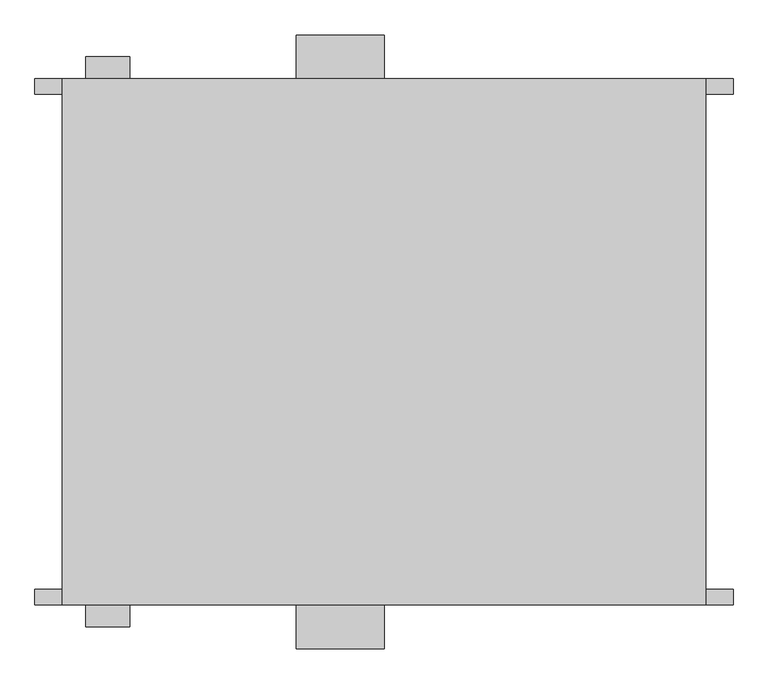
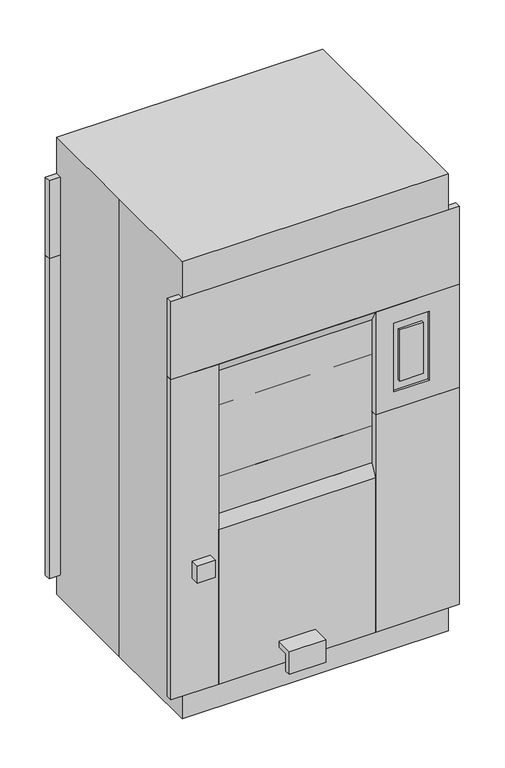
"""IFC4 building model written with IfcOpenShell, lengths in millimetres: proxy geometry, S0960 - Washer-Disinfector, STM, 2 DO, RCSD1WLL, 26x24x24 Cham : S0960 - Washer-Disinfector, STM, 2 DO, RCSD1WLL, 26x24x24 Cham."""

from ifc_helpers import new_model, si_unit, frame, origin, place, context, project, spatial, polyline, outline, extrude, faceted_brep, source, transform, mapped, element, save


def specialty_equipment_aeb0d0a3(model_context):
    return source(origin(), model_context, "Body", "SolidModel", [
        extrude(outline(polyline([(-457.2, 101.6), (-457.2, 787.4), (-430.2125, 838.2), (-430.2125, 101.6), (-457.2, 101.6)])), frame((-406.4, 0.0, 0.0), z_axis=(1.0, 0.0, 0.0), x_axis=(0.0, 1.0, 0.0)), (0.0, 0.0, 1.0), 660.4),
        extrude(outline(polyline([(-430.2125, 1524.0), (-430.2125, 1473.2), (-457.2, 1524.0), (-430.2125, 1524.0)])), frame((-406.4, 0.0, 0.0), z_axis=(1.0, 0.0, 0.0), x_axis=(0.0, 1.0, 0.0)), (0.0, 0.0, 1.0), 660.4),
        faceted_brep([(606.425, -457.2, 1524.0), (254.0, -457.2, 1524.0), (254.0, -457.2, 1066.8), (606.425, -457.2, 1066.8), (479.425, -457.2, 1447.8), (479.425, -457.2, 1143.0), (330.2, -457.2, 1143.0), (330.2, -457.2, 1447.8), (454.025, -457.2, 1409.7), (355.6, -457.2, 1409.7), (355.6, -457.2, 1181.1), (454.025, -457.2, 1181.1), (606.425, -430.2125, 1524.0), (606.425, -430.2125, 1066.8), (254.0, -430.2125, 1066.8), (254.0, -430.2125, 1524.0), (479.425, -448.0871048, 1447.8), (330.2, -448.0871048, 1447.8), (330.2, -448.0871048, 1143.0), (479.425, -448.0871048, 1143.0), (454.025, -448.0871048, 1409.7), (454.025, -448.0871048, 1181.1), (355.6, -448.0871048, 1181.1), (355.6, -448.0871048, 1409.7)], [[[0, 1, 2, 3], [4, 5, 6, 7]], [[8, 9, 10, 11]], [[12, 13, 14, 15]], [[0, 12, 15, 1]], [[1, 15, 14, 2]], [[2, 14, 13, 3]], [[3, 13, 12, 0]], [[16, 17, 18, 19], [20, 21, 22, 23]], [[16, 4, 7, 17]], [[17, 7, 6, 18]], [[18, 6, 5, 19]], [[19, 5, 4, 16]], [[20, 8, 11, 21]], [[21, 11, 10, 22]], [[22, 10, 9, 23]], [[23, 9, 8, 20]]]),
        extrude(outline(polyline([(606.425, 457.2), (606.425, 430.2125), (254.0, 430.2125), (254.0, 457.2), (606.425, 457.2)])), frame((0.0, 0.0, 101.6), z_axis=(0.0, 0.0, 1.0), x_axis=(1.0, 0.0, 0.0)), (0.0, 0.0, 1.0), 965.2),
        extrude(outline(polyline([(-406.4, 457.2), (-406.4, 430.2125), (-606.425, 430.2125), (-606.425, 457.2), (-406.4, 457.2)])), frame((0.0, 0.0, 101.6), z_axis=(0.0, 0.0, 1.0), x_axis=(1.0, 0.0, 0.0)), (0.0, 0.0, 1.0), 1422.4),
        extrude(outline(polyline([(606.425, 457.2), (606.425, 430.2125), (-606.425, 430.2125), (-606.425, 457.2), (606.425, 457.2)])), frame((0.0, 0.0, 1524.0), z_axis=(0.0, 0.0, 1.0), x_axis=(1.0, 0.0, 0.0)), (0.0, 0.0, 1.0), 346.075),
        extrude(outline(polyline([(-533.4, 203.2), (-457.2, 203.2), (-457.2, 177.8), (-508.0, 177.8), (-508.0, 101.6), (-533.4, 101.6), (-533.4, 203.2)])), frame((-152.4, 0.0, 0.0), z_axis=(1.0, 0.0, 0.0), x_axis=(0.0, 1.0, 0.0)), (0.0, 0.0, 1.0), 152.4),
        extrude(outline(polyline([(-517.7182221, -495.3), (-517.7182221, -457.2), (-441.5182221, -457.2), (-441.5182221, -495.3), (-517.7182221, -495.3)])), frame((0.0, 0.0, 611.2734951), z_axis=(0.0, 0.0, 1.0), x_axis=(1.0, 0.0, 0.0)), (0.0, 0.0, 1.0), 76.2),
        extrude(outline(polyline([(254.0, -457.2), (254.0, -430.2125), (606.425, -430.2125), (606.425, -457.2), (254.0, -457.2)])), frame((0.0, 0.0, 101.6), z_axis=(0.0, 0.0, 1.0), x_axis=(1.0, 0.0, 0.0)), (0.0, 0.0, 1.0), 965.2),
        extrude(outline(polyline([(-606.425, -457.2), (-606.425, -430.2125), (-406.4, -430.2125), (-406.4, -457.2), (-606.425, -457.2)])), frame((0.0, 0.0, 101.6), z_axis=(0.0, 0.0, 1.0), x_axis=(1.0, 0.0, 0.0)), (0.0, 0.0, 1.0), 1422.4),
        extrude(outline(polyline([(-606.425, -457.2), (-606.425, -430.2125), (606.425, -430.2125), (606.425, -457.2), (-606.425, -457.2)])), frame((0.0, 0.0, 1524.0), z_axis=(0.0, 0.0, 1.0), x_axis=(1.0, 0.0, 0.0)), (0.0, 0.0, 1.0), 346.075),
        extrude(outline(polyline([(533.4, 203.2), (533.4, 101.6), (508.0, 101.6), (508.0, 177.8), (457.2, 177.8), (457.2, 203.2), (533.4, 203.2)])), frame((-152.4, 0.0, 0.0), z_axis=(1.0, 0.0, 0.0), x_axis=(0.0, 1.0, 0.0)), (0.0, 0.0, 1.0), 152.4),
        extrude(outline(polyline([(-441.5182221, 495.3), (-441.5182221, 457.2), (-517.7182221, 457.2), (-517.7182221, 495.3), (-441.5182221, 495.3)])), frame((0.0, 0.0, 611.2734951), z_axis=(0.0, 0.0, 1.0), x_axis=(1.0, 0.0, 0.0)), (0.0, 0.0, 1.0), 76.2),
        extrude(outline(polyline([(430.2125, 101.6), (430.2125, 838.2), (457.2, 787.4), (457.2, 101.6), (430.2125, 101.6)])), frame((-406.4, 0.0, 0.0), z_axis=(1.0, 0.0, 0.0), x_axis=(0.0, 1.0, 0.0)), (0.0, 0.0, 1.0), 660.4),
        extrude(outline(polyline([(457.2, 1524.0), (430.2125, 1473.2), (430.2125, 1524.0), (457.2, 1524.0)])), frame((-406.4, 0.0, 0.0), z_axis=(1.0, 0.0, 0.0), x_axis=(0.0, 1.0, 0.0)), (0.0, 0.0, 1.0), 660.4),
        faceted_brep([(606.425, 457.2, 1524.0), (606.425, 457.2, 1066.8), (254.0, 457.2, 1066.8), (254.0, 457.2, 1524.0), (330.2, 457.2, 1447.8), (330.2, 457.2, 1143.0), (479.425, 457.2, 1143.0), (479.425, 457.2, 1447.8), (454.025, 457.2, 1181.1), (355.6, 457.2, 1181.1), (355.6, 457.2, 1409.7), (454.025, 457.2, 1409.7), (606.425, 430.2125, 1524.0), (254.0, 430.2125, 1524.0), (254.0, 430.2125, 1066.8), (606.425, 430.2125, 1066.8), (479.425, 448.0871048, 1447.8), (479.425, 448.0871048, 1143.0), (330.2, 448.0871048, 1143.0), (330.2, 448.0871048, 1447.8), (454.025, 448.0871048, 1409.7), (355.6, 448.0871048, 1409.7), (355.6, 448.0871048, 1181.1), (454.025, 448.0871048, 1181.1)], [[[0, 1, 2, 3], [4, 5, 6, 7]], [[8, 9, 10, 11]], [[12, 13, 14, 15]], [[3, 13, 12, 0]], [[2, 14, 13, 3]], [[1, 15, 14, 2]], [[0, 12, 15, 1]], [[16, 17, 18, 19], [20, 21, 22, 23]], [[19, 4, 7, 16]], [[18, 5, 4, 19]], [[17, 6, 5, 18]], [[16, 7, 6, 17]], [[23, 8, 11, 20]], [[22, 9, 8, 23]], [[21, 10, 9, 22]], [[20, 11, 10, 21]]]),
        extrude(outline(polyline([(254.0, 430.2125), (254.0, -430.2125), (-406.4, -430.2125), (-406.4, 430.2125), (254.0, 430.2125)])), frame((0.0, 0.0, 838.2), z_axis=(0.0, 0.0, 1.0), x_axis=(1.0, 0.0, 0.0)), (0.0, 0.0, 1.0), 635.0),
        extrude(outline(polyline([(0.0, 555.625), (1870.075, 555.625), (1870.075, -555.625), (0.0, -555.625), (0.0, 555.625)]), holes=[polyline([(838.2, -406.4), (996.95, -406.4), (996.95, 254.0), (838.2, 254.0), (838.2, -406.4)]), polyline([(1473.2, 254.0), (1320.8, 254.0), (1320.8, -406.4), (1473.2, -406.4), (1473.2, 254.0)]), polyline([(1314.45, 254.0), (1162.05, 254.0), (1162.05, -406.4), (1314.45, -406.4), (1314.45, 254.0)]), polyline([(1155.7, 254.0), (1003.3, 254.0), (1003.3, -406.4), (1155.7, -406.4), (1155.7, 254.0)])]), frame((0.0, -430.2125, 0.0), z_axis=(0.0, 1.0, 0.0), x_axis=(0.0, 0.0, 1.0)), (0.0, 0.0, 1.0), 860.425),
        faceted_brep([(-558.8, -457.2, 2032.0), (558.8, -457.2, 2032.0), (558.8, 457.2, 2032.0), (-558.8, 457.2, 2032.0), (-558.8, 0.0, 2032.0), (-558.8, -457.2, 0.0), (-558.8, 0.0, 0.0), (-558.8, 457.2, 0.0), (558.8, 457.2, 0.0), (558.8, -457.2, 0.0), (-406.4, 457.2, 1524.0), (-406.4, 457.2, 787.4), (254.0, 457.2, 787.4), (254.0, 457.2, 1524.0), (330.2, 457.2, 1447.8), (330.2, 457.2, 1143.0), (479.425, 457.2, 1143.0), (479.425, 457.2, 1447.8), (454.025, 457.2, 1181.1), (355.6, 457.2, 1181.1), (355.6, 457.2, 1409.7), (454.025, 457.2, 1409.7), (254.0, -457.2, 1524.0), (254.0, -457.2, 787.4), (-406.4, -457.2, 787.4), (-406.4, -457.2, 1524.0), (479.425, -457.2, 1447.8), (479.425, -457.2, 1143.0), (330.2, -457.2, 1143.0), (330.2, -457.2, 1447.8), (454.025, -457.2, 1409.7), (355.6, -457.2, 1409.7), (355.6, -457.2, 1181.1), (454.025, -457.2, 1181.1), (254.0, 430.2125, 1473.2), (254.0, 430.2125, 838.2), (-406.4, 430.2125, 838.2), (-406.4, 430.2125, 1473.2), (-406.4, 455.6125, 1524.0), (-406.4, 455.6125, 1521.0117647), (254.0, 455.6125, 1521.0117647), (254.0, 455.6125, 1524.0), (254.0, 455.6125, 787.4), (254.0, 455.6125, 790.3882353), (-406.4, 455.6125, 790.3882353), (-406.4, 455.6125, 787.4), (479.425, 448.0871048, 1447.8), (479.425, 448.0871048, 1143.0), (330.2, 448.0871048, 1143.0), (330.2, 448.0871048, 1447.8), (454.025, 448.0871048, 1409.7), (355.6, 448.0871048, 1409.7), (355.6, 448.0871048, 1181.1), (454.025, 448.0871048, 1181.1), (254.0, -430.2125, 1473.2), (-406.4, -430.2125, 1473.2), (-406.4, -430.2125, 838.2), (254.0, -430.2125, 838.2), (479.425, -448.0871048, 1447.8), (330.2, -448.0871048, 1447.8), (330.2, -448.0871048, 1143.0), (479.425, -448.0871048, 1143.0), (454.025, -448.0871048, 1409.7), (454.025, -448.0871048, 1181.1), (355.6, -448.0871048, 1181.1), (355.6, -448.0871048, 1409.7)], [[[0, 1, 2, 3, 4]], [[5, 6, 7, 8, 9]], [[4, 6, 5, 0]], [[3, 7, 6, 4]], [[2, 8, 7, 3], [10, 11, 12, 13], [14, 15, 16, 17]], [[18, 19, 20, 21]], [[1, 9, 8, 2]], [[0, 5, 9, 1], [22, 23, 24, 25], [26, 27, 28, 29]], [[30, 31, 32, 33]], [[34, 35, 36, 37]], [[38, 39, 40, 41]], [[42, 43, 44, 45]], [[37, 38, 41, 34]], [[36, 45, 44, 11, 10, 39, 38, 37]], [[35, 42, 45, 36]], [[34, 41, 40, 13, 12, 43, 42, 35]], [[10, 13, 40, 39]], [[44, 43, 12, 11]], [[46, 47, 48, 49], [50, 51, 52, 53]], [[49, 14, 17, 46]], [[48, 15, 14, 49]], [[47, 16, 15, 48]], [[46, 17, 16, 47]], [[53, 18, 21, 50]], [[52, 19, 18, 53]], [[51, 20, 19, 52]], [[50, 21, 20, 51]], [[54, 55, 56, 57]], [[54, 22, 25, 55]], [[55, 25, 24, 56]], [[56, 24, 23, 57]], [[57, 23, 22, 54]], [[58, 59, 60, 61], [62, 63, 64, 65]], [[58, 26, 29, 59]], [[59, 29, 28, 60]], [[60, 28, 27, 61]], [[61, 27, 26, 58]], [[62, 30, 33, 63]], [[63, 33, 32, 64]], [[64, 32, 31, 65]], [[65, 31, 30, 62]]]),
    ])


if __name__ == "__main__":
    model = new_model("IFC4")
    model_context = context("Model", 3, world=origin())
    ifc_project = project(units=[si_unit("LENGTHUNIT", "METRE", prefix="MILLI")], contexts=[model_context])
    site = spatial("IfcSite", under=ifc_project)
    building = spatial("IfcBuilding", under=site)
    placement = place(None, origin())
    specialty_equipment_shape = specialty_equipment_aeb0d0a3(model_context)
    element("IfcBuildingElementProxy", 1, Name="S0960 - Washer-Disinfector, STM, 2 DO, RCSD1WLL, 26x24x24 Cham : S0960 - Washer-Disinfector, STM, 2 DO, RCSD1WLL, 26x24x24 Cham", ObjectType="S0960 - Washer-Disinfector, STM, 2 DO, RCSD1WLL, 26x24x24 Cham : S0960 - Washer-Disinfector, STM, 2 DO, RCSD1WLL, 26x24x24 Cham", at=placement, inside=building, context=model_context, shape_type="MappedRepresentation", body=[
        mapped(specialty_equipment_shape, transform((0.0, 0.0, 0.0), x_axis=(1.0, 0.0, 0.0), y_axis=(0.0, 1.0, 0.0), z_axis=(0.0, 0.0, 1.0))),
    ])
    save(model, "model.ifc")

# Revit data of these elements
# Type "S0960 - Washer-Disinfector, STM, 2 DO, RCSD1WLL, 26x24x24 Cham : S0960 - Washer-Disinfector, STM, 2 DO, RCSD1WLL, 26x24x24 Cham"
#   Watts2 = "0"
#   Watts1 = "7206"
#   Unit_Issue = "EA"
#   UTIL_6_Misc = "E"
#   UTIL_5_NonMedGas = "-"
#   UTIL_4_MiscGas = "A"
#   UTIL_3_MedGas = "D"
#   UTIL_2_Elec = "G"
#   UTIL_1_WaterDrain = "F"
#   Nomenclature = "Washer/Disinfector,STM,2DO,RCSD1WLL,26X24X24 Cham"
#   NSN = "6530"
#   Location [instance default] = ""
#   JSN = "S0960"
#   Fund_Source_VA = "-"
#   Fund_Source_Navy = "-"
#   Fund_Source_Army = "-"
#   Fund_Source_AF = "-"
#   ELEC_Volts2 = "0"
#   ELEC_Volts1 = "208"
#   ELEC_Phase2 = "0"
#   ELEC_Phase1 = "3"
#   ELEC_HertzSwitch = "-1"
#   ELEC_HertzDependent = "0"
#   ELEC_Hertz = "50/60"
#   ELEC_Amps2 = "0"
#   ELEC_Amps1 = "20"
#   DetailDescription = "A recessed mounted (through one wall), double door (vertical sliding with tempered glass window), multi-level, mechanical, washer/disinfector, minimum chamber size 26X24X24, utilizing facility supplied steam. The unit is controlled by a microcomputer that monitors and controls all unit operations and functions and provides both audible and visual indications of deviations. A printer-recorder documents and records each cycle performance. Processing cycles are pre-programmed with pre-wash, wash/cleaning, rinse, and thermal rinse/disinfection. For use in health care facilities and laboratories where reusable items (instruments, utensils, anesthesia/respiratory goods, and glassware) are handled for decontamination purposes. This unit is not a substitute for terminal sterilization. Unit available with manual or power door, various electrical configurations, options, and accessories. Price based upon power door, 208V, 3-phase, with various options."
#   CAT_VA = "C"
#   CAT_Navy = "C"
#   CAT_IHS = "-"
#   CAT_Army = "A"
#   CAT_AF = "C"
#   BTUperhour = "0"
#   Weight_IP = 1200
#   DIM_Width_IP = 3' - 8"
#   DIM_Height_IP = 6' - 8"
#   DIM_Depth_IP = 3' - 0"
# Element 1 (IfcBuildingElementProxy, "S0960 - Washer-Disinfector, STM, 2 DO, RCSD1WLL, 26x24x24 Cham : S0960 - Washer-Disinfector, STM, 2 DO, RCSD1WLL, 26x24x24 Cham")
#   Materials on its faces: "EquipSpace", "Glass"
# Materials
#   "EquipSpace": class "Unassigned", colour RGB 221 217 195, transparency 0.5
#   "Glass": class "Glass", colour RGB 0 128 192, transparency 0.75
